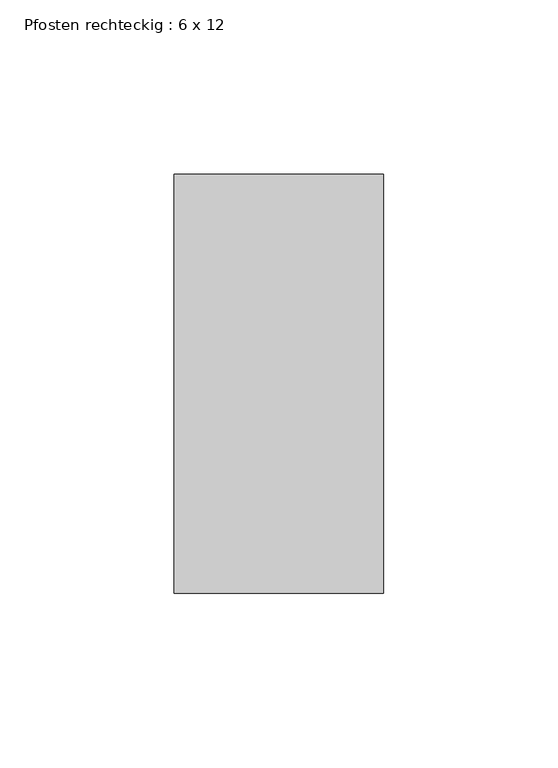
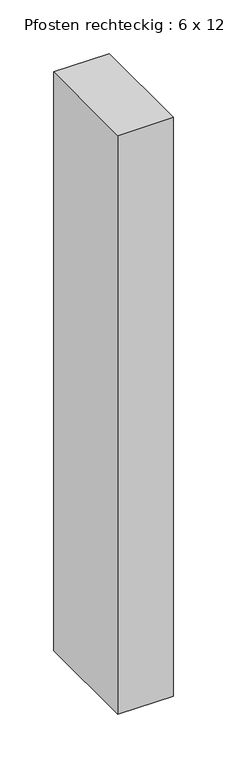
"""IFC4 building model written with IfcOpenShell, lengths in millimetres: member geometry, Pfosten rechteckig : 6 x 12."""

import ifcopenshell
import ifcopenshell.guid

model = None  # the IFC model being written
_history = None  # IfcOwnerHistory: only IFC2X3 demands one
_inside = {}  # id of a spatial element -> (the spatial element, [elements in it])
_under = {}  # id of a project, library or spatial element -> (it, [spatial elements below it])
_declared = {}  # id of a project -> (the project, [libraries it declares])
_typed = {}  # id of a type object -> (the type object, [elements of that type])
_made_of = {}  # id of a material, layer set ... -> (it, [elements and type objects made of it])


def new_model(schema):
    """Start an empty IFC model of exactly this schema.

    Asked for "IFC4X3", IfcOpenShell would pick the latest addendum, in which some entities
    have other attributes; the version numbers below select the first issue.
    IFC2X3 requires an IfcOwnerHistory on every rooted entity: one is made here for all.
    """
    global model, _history
    if schema == "IFC4X3":
        model = ifcopenshell.file(schema_version=(4, 3, 0, 0))
    else:
        model = ifcopenshell.file(schema=schema)
    _inside.clear()
    _under.clear()
    _declared.clear()
    _typed.clear()
    _made_of.clear()
    _history = None
    if model.schema == "IFC2X3":
        org = make("IfcOrganization", Name="unknown")
        user = make(
            "IfcPersonAndOrganization",
            ThePerson=make("IfcPerson", FamilyName="unknown"),
            TheOrganization=org,
        )
        app = make(
            "IfcApplication",
            ApplicationDeveloper=org,
            Version="unknown",
            ApplicationFullName="unknown",
            ApplicationIdentifier="unknown",
        )
        _history = make(
            "IfcOwnerHistory",
            OwningUser=user,
            OwningApplication=app,
            ChangeAction="ADDED",
            CreationDate=0,
        )
    return model


def make(cls, **values):
    """One entity of the class cls with the attributes given. An attribute that is None is left unset."""
    return model.create_entity(
        cls, **{name: value for name, value in values.items() if value is not None}
    )


def rooted(cls, **values):
    """An entity with a GlobalId (a new one), such as an element, a storey or a relation."""
    return make(cls, GlobalId=ifcopenshell.guid.new(), OwnerHistory=_history, **values)


def si_unit(unit_type, name, prefix=None):
    """IfcSIUnit, for example si_unit("LENGTHUNIT", "METRE", prefix="MILLI")."""
    return make("IfcSIUnit", UnitType=unit_type, Prefix=prefix, Name=name)


def assignment(units):
    """IfcUnitAssignment: the units of a project."""
    return None if units is None else make("IfcUnitAssignment", Units=units)


def point(xyz):
    """IfcCartesianPoint."""
    return None if xyz is None else make("IfcCartesianPoint", Coordinates=xyz)


def direction(xyz):
    """IfcDirection."""
    return None if xyz is None else make("IfcDirection", DirectionRatios=xyz)


def frame(location, z_axis=None, x_axis=None):
    """IfcAxis2Placement3D, a coordinate frame: its origin and axes. An axis left out is left unset."""
    return make(
        "IfcAxis2Placement3D",
        Location=point(location),
        Axis=direction(z_axis),
        RefDirection=direction(x_axis),
    )


def origin():
    """The frame at (0, 0, 0) with its axes left unset."""
    return frame((0.0, 0.0, 0.0))


def place(relative_to, where):
    """IfcLocalPlacement: puts the frame where relative to a parent placement (None: the world)."""
    return make(
        "IfcLocalPlacement", PlacementRelTo=relative_to, RelativePlacement=where
    )


def context(
    kind, dimensions, precision=None, world=None, true_north=None, identifier=None
):
    """IfcGeometricRepresentationContext, for example the 3D "Model" context."""
    return make(
        "IfcGeometricRepresentationContext",
        ContextIdentifier=identifier,
        ContextType=kind,
        CoordinateSpaceDimension=dimensions,
        Precision=precision,
        WorldCoordinateSystem=world,
        TrueNorth=true_north,
    )


def project(units=None, contexts=None):
    """IfcProject with its units and contexts."""
    return rooted(
        "IfcProject",
        Name="project",
        RepresentationContexts=contexts,
        UnitsInContext=assignment(units),
    )


def spatial(cls, under=None, at=None, **own):
    """A site, building, storey or space (cls), placed at a placement, below another one or the project."""
    s = rooted(cls, ObjectPlacement=at, **own)
    if under is not None:
        _under.setdefault(under.id(), (under, []))[1].append(s)
    return s


def polyline(points):
    """IfcPolyline through the points."""
    return make("IfcPolyline", Points=[point(p) for p in points])


def outline(outer, holes=None, kind="AREA"):
    """IfcArbitraryClosedProfileDef: a profile drawn as a closed curve; with holes, ...WithVoids."""
    if holes is None:
        return make("IfcArbitraryClosedProfileDef", ProfileType=kind, OuterCurve=outer)
    return make(
        "IfcArbitraryProfileDefWithVoids",
        ProfileType=kind,
        OuterCurve=outer,
        InnerCurves=holes,
    )


def extrude(swept, where, along, depth):
    """IfcExtrudedAreaSolid: the profile swept, set in the frame where, extruded along a direction by depth."""
    return make(
        "IfcExtrudedAreaSolid",
        SweptArea=swept,
        Position=where,
        ExtrudedDirection=direction(along),
        Depth=depth,
    )


def shape(context_of_items, identifier, shape_type, items):
    """IfcShapeRepresentation: the items that make up one representation, for example the "Body"."""
    return make(
        "IfcShapeRepresentation",
        ContextOfItems=context_of_items,
        RepresentationIdentifier=identifier,
        RepresentationType=shape_type,
        Items=items,
    )


def source(mapping_origin, context_of_items, identifier, shape_type, items):
    """IfcRepresentationMap: a shape defined once, which mapped items show again and again."""
    return make(
        "IfcRepresentationMap",
        MappingOrigin=mapping_origin,
        MappedRepresentation=shape(context_of_items, identifier, shape_type, items),
    )


def transform(
    local_origin,
    x_axis=None,
    y_axis=None,
    z_axis=None,
    scale=None,
    scale2=None,
    scale3=None,
    uniform=True,
):
    """IfcCartesianTransformationOperator3D, or its non-uniform kind. x_axis, y_axis, z_axis: its Axis1, 2, 3."""
    if uniform:
        return make(
            "IfcCartesianTransformationOperator3D",
            Axis1=direction(x_axis),
            Axis2=direction(y_axis),
            LocalOrigin=point(local_origin),
            Scale=scale,
            Axis3=direction(z_axis),
        )
    return make(
        "IfcCartesianTransformationOperator3DnonUniform",
        Axis1=direction(x_axis),
        Axis2=direction(y_axis),
        LocalOrigin=point(local_origin),
        Scale=scale,
        Axis3=direction(z_axis),
        Scale2=scale2,
        Scale3=scale3,
    )


def mapped(mapping_source, mapping_target):
    """IfcMappedItem: shows the shape of a source again, moved by a transform."""
    return make(
        "IfcMappedItem", MappingSource=mapping_source, MappingTarget=mapping_target
    )


def made_of(thing, what):
    """Note that an element or type object is made of a material, layer set ...; save() writes the relation."""
    if what is not None:
        _made_of.setdefault(what.id(), (what, []))[1].append(thing)
    return thing


def element(
    cls,
    number,
    at=None,
    inside=None,
    cuts=None,
    type_object=None,
    material=None,
    context=None,
    identifier="Body",
    shape_type=None,
    held_by="IfcProductDefinitionShape",
    body=None,
    shapes=None,
    **own,
):
    """One element of the class cls, such as IfcWall. Its Tag is "e" and its number.

    at: its placement. inside: the storey or other place that contains it. cuts: it is an
    opening in that element (IfcRelVoidsElement). A single representation is given by context,
    identifier, shape_type and body (its items); several are given by shapes. held_by: the class
    of the entity that holds the representations. save() writes the other relations.
    """
    e = rooted(cls, Tag="e%d" % number, ObjectPlacement=at, **own)
    if body is not None:
        shapes = [shape(context, identifier, shape_type, body)]
    if shapes is not None:
        e.Representation = make(held_by, Representations=shapes)
    if inside is not None:
        _inside.setdefault(inside.id(), (inside, []))[1].append(e)
    if cuts is not None:
        rooted(
            "IfcRelVoidsElement", RelatingBuildingElement=cuts, RelatedOpeningElement=e
        )
    if type_object is not None:
        _typed.setdefault(type_object.id(), (type_object, []))[1].append(e)
    return made_of(e, material)


def aggregate(whole, parts):
    """IfcRelAggregates: a whole, such as a stair, and the parts it consists of."""
    return rooted("IfcRelAggregates", RelatingObject=whole, RelatedObjects=parts)


def save(model, path):
    """Write the relations noted so far, then the file.

    IfcRelAggregates (storeys below a building ...), IfcRelContainedInSpatialStructure (elements
    in a storey), IfcRelDefinesByType, IfcRelAssociatesMaterial and IfcRelDeclares: one each for
    every whole, place, type object, material and project.
    """
    for whole, parts in _under.values():
        aggregate(whole, parts)
    for where, things in _inside.values():
        rooted(
            "IfcRelContainedInSpatialStructure",
            RelatedElements=things,
            RelatingStructure=where,
        )
    for kind, things in _typed.values():
        rooted("IfcRelDefinesByType", RelatedObjects=things, RelatingType=kind)
    for what, things in _made_of.values():
        rooted("IfcRelAssociatesMaterial", RelatedObjects=things, RelatingMaterial=what)
    for by, libraries in _declared.values():
        rooted("IfcRelDeclares", RelatingContext=by, RelatedDefinitions=libraries)
    model.write(path)


def pfosten_rechteckig_6_x_12_97c23e68(model_context):
    return source(origin(), model_context, "Body", "SweptSolid", [
        extrude(outline(polyline([(0.0, 60.0), (0.0, -60.0), (-60.0, -60.0), (-60.0, 60.0), (0.0, 60.0)])), frame((0.0, 0.0, -660.287322), z_axis=(0.0, 0.0, 1.0), x_axis=(1.0, 0.0, 0.0)), (0.0, 0.0, 1.0), 660.287322),
    ])


if __name__ == "__main__":
    model = new_model("IFC4")
    model_context = context("Model", 3, world=origin())
    ifc_project = project(units=[si_unit("LENGTHUNIT", "METRE", prefix="MILLI")], contexts=[model_context])
    site = spatial("IfcSite", under=ifc_project)
    building = spatial("IfcBuilding", under=site)
    placement = place(None, origin())
    pfosten_rechteckig_6_x_12_shape = pfosten_rechteckig_6_x_12_97c23e68(model_context)
    element("IfcMember", 1, ObjectType="Pfosten rechteckig : 6 x 12", at=placement, inside=building, context=model_context, shape_type="MappedRepresentation", body=[
        mapped(pfosten_rechteckig_6_x_12_shape, transform((0.0, 0.0, 0.0), x_axis=(1.0, 0.0, 0.0), y_axis=(0.0, 1.0, 0.0), z_axis=(0.0, 0.0, 1.0))),
    ])
    save(model, "model.ifc")

# Revit data of these elements
# Type "Pfosten rechteckig : 6 x 12"
#   built-in parameter 1007304 = 0.393701 (stored number, unit not read)
#   built-in parameter 1007301 = 0.0984252 (stored number, unit not read)
#   built-in parameter 1007300 = 0.0984252 (stored number, unit not read)
# Element 1 (IfcMember, "Pfosten rechteckig : 6 x 12")
#   Materials on its faces: "Metall - verzinkt"
# Materials
#   "Metall - verzinkt": class "Allgemeines", colour RGB 200 200 200, transparency 0, Cost = 0
